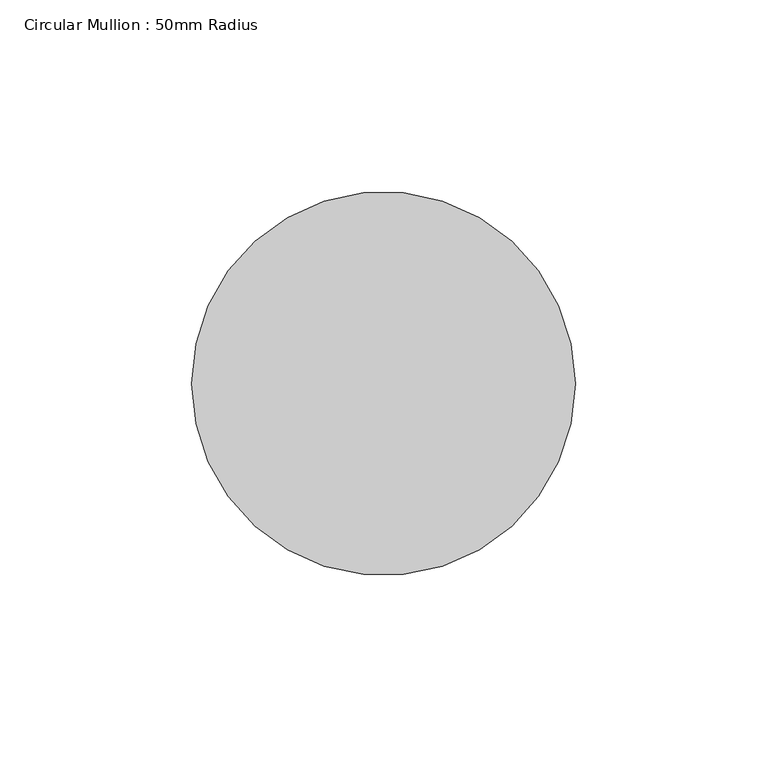
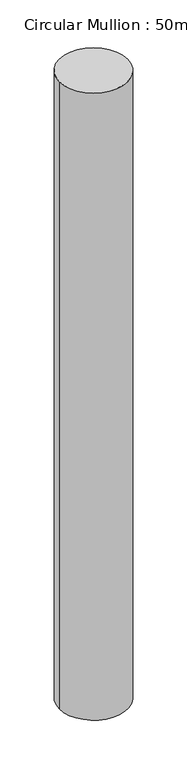
"""IFC4 building model written with IfcOpenShell, lengths in millimetres: member geometry, Circular Mullion : 50mm Radius."""

from ifc_helpers import new_model, si_unit, point, frame, origin, origin_2d, place, context, project, spatial, circle_curve, trimmed, segment, composite_curve, outline, extrude, source, transform, mapped, element, save


def circular_mullion_50mm_radius_a89d009e(model_context):
    return source(origin(), model_context, "Body", "SweptSolid", [
        extrude(outline(composite_curve([segment(trimmed(circle_curve(origin_2d(), 50.0), [point((50.0, 0.0))], [point((-50.0, 0.0))], False, "CARTESIAN"), True, "CONTINUOUS"), segment(trimmed(circle_curve(origin_2d(), 50.0), [point((-50.0, 0.0))], [point((50.0, 0.0))], False, "CARTESIAN"), True, "CONTINUOUS")], self_intersect=False)), frame((0.0, 0.0, -969.3449188), z_axis=(0.0, 0.0, 1.0), x_axis=(1.0, 0.0, 0.0)), (0.0, 0.0, 1.0), 969.3449188),
    ])


if __name__ == "__main__":
    model = new_model("IFC4")
    model_context = context("Model", 3, world=origin())
    ifc_project = project(units=[si_unit("LENGTHUNIT", "METRE", prefix="MILLI")], contexts=[model_context])
    site = spatial("IfcSite", under=ifc_project)
    building = spatial("IfcBuilding", under=site)
    placement = place(None, origin())
    circular_mullion_50mm_radius_shape = circular_mullion_50mm_radius_a89d009e(model_context)
    element("IfcMember", 1, ObjectType="Circular Mullion : 50mm Radius", at=placement, inside=building, context=model_context, shape_type="MappedRepresentation", body=[
        mapped(circular_mullion_50mm_radius_shape, transform((0.0, 0.0, 0.0), x_axis=(1.0, 0.0, 0.0), y_axis=(0.0, 1.0, 0.0), z_axis=(0.0, 0.0, 1.0))),
    ])
    save(model, "model.ifc")

# Revit data of these elements
# Type "Circular Mullion : 50mm Radius"
#   built-in parameter 1007350 = 0.164042 (stored number, unit not read)
# Element 1 (IfcMember, "Circular Mullion : 50mm Radius")
#   Materials on its faces: "Aluminium"
# Materials
#   "Aluminium": class "Metal", colour RGB 247 247 247, transparency 0, Description = "Aluminium 6061", Cost = 0
